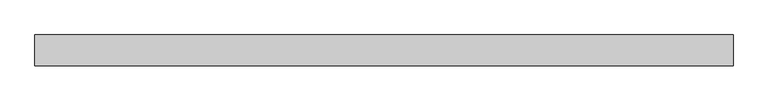
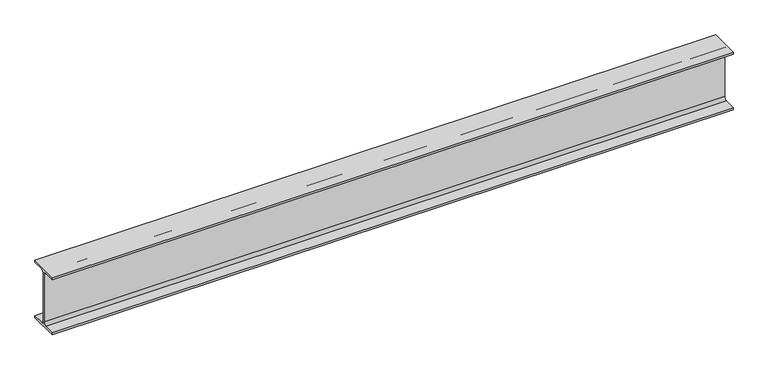
"""IFC4 building model written with IfcOpenShell, lengths in millimetres: beam geometry, 0912_Steel Framing_H-KSD3502 : H_SB_ASB_H-250x125x6x9."""

import ifcopenshell
import ifcopenshell.guid

model = None  # the IFC model being written
_history = None  # IfcOwnerHistory: only IFC2X3 demands one
_inside = {}  # id of a spatial element -> (the spatial element, [elements in it])
_under = {}  # id of a project, library or spatial element -> (it, [spatial elements below it])
_declared = {}  # id of a project -> (the project, [libraries it declares])
_typed = {}  # id of a type object -> (the type object, [elements of that type])
_made_of = {}  # id of a material, layer set ... -> (it, [elements and type objects made of it])


def new_model(schema):
    """Start an empty IFC model of exactly this schema.

    Asked for "IFC4X3", IfcOpenShell would pick the latest addendum, in which some entities
    have other attributes; the version numbers below select the first issue.
    IFC2X3 requires an IfcOwnerHistory on every rooted entity: one is made here for all.
    """
    global model, _history
    if schema == "IFC4X3":
        model = ifcopenshell.file(schema_version=(4, 3, 0, 0))
    else:
        model = ifcopenshell.file(schema=schema)
    _inside.clear()
    _under.clear()
    _declared.clear()
    _typed.clear()
    _made_of.clear()
    _history = None
    if model.schema == "IFC2X3":
        org = make("IfcOrganization", Name="unknown")
        user = make(
            "IfcPersonAndOrganization",
            ThePerson=make("IfcPerson", FamilyName="unknown"),
            TheOrganization=org,
        )
        app = make(
            "IfcApplication",
            ApplicationDeveloper=org,
            Version="unknown",
            ApplicationFullName="unknown",
            ApplicationIdentifier="unknown",
        )
        _history = make(
            "IfcOwnerHistory",
            OwningUser=user,
            OwningApplication=app,
            ChangeAction="ADDED",
            CreationDate=0,
        )
    return model


def make(cls, **values):
    """One entity of the class cls with the attributes given. An attribute that is None is left unset."""
    return model.create_entity(
        cls, **{name: value for name, value in values.items() if value is not None}
    )


def rooted(cls, **values):
    """An entity with a GlobalId (a new one), such as an element, a storey or a relation."""
    return make(cls, GlobalId=ifcopenshell.guid.new(), OwnerHistory=_history, **values)


def si_unit(unit_type, name, prefix=None):
    """IfcSIUnit, for example si_unit("LENGTHUNIT", "METRE", prefix="MILLI")."""
    return make("IfcSIUnit", UnitType=unit_type, Prefix=prefix, Name=name)


def assignment(units):
    """IfcUnitAssignment: the units of a project."""
    return None if units is None else make("IfcUnitAssignment", Units=units)


def point(xyz):
    """IfcCartesianPoint."""
    return None if xyz is None else make("IfcCartesianPoint", Coordinates=xyz)


def direction(xyz):
    """IfcDirection."""
    return None if xyz is None else make("IfcDirection", DirectionRatios=xyz)


def frame(location, z_axis=None, x_axis=None):
    """IfcAxis2Placement3D, a coordinate frame: its origin and axes. An axis left out is left unset."""
    return make(
        "IfcAxis2Placement3D",
        Location=point(location),
        Axis=direction(z_axis),
        RefDirection=direction(x_axis),
    )


def frame_2d(location, x_axis=None):
    """IfcAxis2Placement2D, a coordinate frame in the plane: its origin and x axis."""
    return make(
        "IfcAxis2Placement2D", Location=point(location), RefDirection=direction(x_axis)
    )


def origin():
    """The frame at (0, 0, 0) with its axes left unset."""
    return frame((0.0, 0.0, 0.0))


def place(relative_to, where):
    """IfcLocalPlacement: puts the frame where relative to a parent placement (None: the world)."""
    return make(
        "IfcLocalPlacement", PlacementRelTo=relative_to, RelativePlacement=where
    )


def context(
    kind, dimensions, precision=None, world=None, true_north=None, identifier=None
):
    """IfcGeometricRepresentationContext, for example the 3D "Model" context."""
    return make(
        "IfcGeometricRepresentationContext",
        ContextIdentifier=identifier,
        ContextType=kind,
        CoordinateSpaceDimension=dimensions,
        Precision=precision,
        WorldCoordinateSystem=world,
        TrueNorth=true_north,
    )


def project(units=None, contexts=None):
    """IfcProject with its units and contexts."""
    return rooted(
        "IfcProject",
        Name="project",
        RepresentationContexts=contexts,
        UnitsInContext=assignment(units),
    )


def spatial(cls, under=None, at=None, **own):
    """A site, building, storey or space (cls), placed at a placement, below another one or the project."""
    s = rooted(cls, ObjectPlacement=at, **own)
    if under is not None:
        _under.setdefault(under.id(), (under, []))[1].append(s)
    return s


def polyline(points):
    """IfcPolyline through the points."""
    return make("IfcPolyline", Points=[point(p) for p in points])


def circle_curve(where, radius):
    """IfcCircle in the frame where."""
    return make("IfcCircle", Position=where, Radius=radius)


def trimmed(basis, trim1, trim2, sense, master):
    """IfcTrimmedCurve: the piece of a basis curve between two trims."""
    return make(
        "IfcTrimmedCurve",
        BasisCurve=basis,
        Trim1=trim1,
        Trim2=trim2,
        SenseAgreement=sense,
        MasterRepresentation=master,
    )


def segment(curve, same_sense, transition):
    """IfcCompositeCurveSegment."""
    return make(
        "IfcCompositeCurveSegment",
        Transition=transition,
        SameSense=same_sense,
        ParentCurve=curve,
    )


def composite_curve(segments, self_intersect=None):
    """IfcCompositeCurve: segments joined end to end."""
    return make("IfcCompositeCurve", Segments=segments, SelfIntersect=self_intersect)


def outline(outer, holes=None, kind="AREA"):
    """IfcArbitraryClosedProfileDef: a profile drawn as a closed curve; with holes, ...WithVoids."""
    if holes is None:
        return make("IfcArbitraryClosedProfileDef", ProfileType=kind, OuterCurve=outer)
    return make(
        "IfcArbitraryProfileDefWithVoids",
        ProfileType=kind,
        OuterCurve=outer,
        InnerCurves=holes,
    )


def extrude(swept, where, along, depth):
    """IfcExtrudedAreaSolid: the profile swept, set in the frame where, extruded along a direction by depth."""
    return make(
        "IfcExtrudedAreaSolid",
        SweptArea=swept,
        Position=where,
        ExtrudedDirection=direction(along),
        Depth=depth,
    )


def shape(context_of_items, identifier, shape_type, items):
    """IfcShapeRepresentation: the items that make up one representation, for example the "Body"."""
    return make(
        "IfcShapeRepresentation",
        ContextOfItems=context_of_items,
        RepresentationIdentifier=identifier,
        RepresentationType=shape_type,
        Items=items,
    )


def source(mapping_origin, context_of_items, identifier, shape_type, items):
    """IfcRepresentationMap: a shape defined once, which mapped items show again and again."""
    return make(
        "IfcRepresentationMap",
        MappingOrigin=mapping_origin,
        MappedRepresentation=shape(context_of_items, identifier, shape_type, items),
    )


def transform(
    local_origin,
    x_axis=None,
    y_axis=None,
    z_axis=None,
    scale=None,
    scale2=None,
    scale3=None,
    uniform=True,
):
    """IfcCartesianTransformationOperator3D, or its non-uniform kind. x_axis, y_axis, z_axis: its Axis1, 2, 3."""
    if uniform:
        return make(
            "IfcCartesianTransformationOperator3D",
            Axis1=direction(x_axis),
            Axis2=direction(y_axis),
            LocalOrigin=point(local_origin),
            Scale=scale,
            Axis3=direction(z_axis),
        )
    return make(
        "IfcCartesianTransformationOperator3DnonUniform",
        Axis1=direction(x_axis),
        Axis2=direction(y_axis),
        LocalOrigin=point(local_origin),
        Scale=scale,
        Axis3=direction(z_axis),
        Scale2=scale2,
        Scale3=scale3,
    )


def mapped(mapping_source, mapping_target):
    """IfcMappedItem: shows the shape of a source again, moved by a transform."""
    return make(
        "IfcMappedItem", MappingSource=mapping_source, MappingTarget=mapping_target
    )


def made_of(thing, what):
    """Note that an element or type object is made of a material, layer set ...; save() writes the relation."""
    if what is not None:
        _made_of.setdefault(what.id(), (what, []))[1].append(thing)
    return thing


def element(
    cls,
    number,
    at=None,
    inside=None,
    cuts=None,
    type_object=None,
    material=None,
    context=None,
    identifier="Body",
    shape_type=None,
    held_by="IfcProductDefinitionShape",
    body=None,
    shapes=None,
    **own,
):
    """One element of the class cls, such as IfcWall. Its Tag is "e" and its number.

    at: its placement. inside: the storey or other place that contains it. cuts: it is an
    opening in that element (IfcRelVoidsElement). A single representation is given by context,
    identifier, shape_type and body (its items); several are given by shapes. held_by: the class
    of the entity that holds the representations. save() writes the other relations.
    """
    e = rooted(cls, Tag="e%d" % number, ObjectPlacement=at, **own)
    if body is not None:
        shapes = [shape(context, identifier, shape_type, body)]
    if shapes is not None:
        e.Representation = make(held_by, Representations=shapes)
    if inside is not None:
        _inside.setdefault(inside.id(), (inside, []))[1].append(e)
    if cuts is not None:
        rooted(
            "IfcRelVoidsElement", RelatingBuildingElement=cuts, RelatedOpeningElement=e
        )
    if type_object is not None:
        _typed.setdefault(type_object.id(), (type_object, []))[1].append(e)
    return made_of(e, material)


def aggregate(whole, parts):
    """IfcRelAggregates: a whole, such as a stair, and the parts it consists of."""
    return rooted("IfcRelAggregates", RelatingObject=whole, RelatedObjects=parts)


def save(model, path):
    """Write the relations noted so far, then the file.

    IfcRelAggregates (storeys below a building ...), IfcRelContainedInSpatialStructure (elements
    in a storey), IfcRelDefinesByType, IfcRelAssociatesMaterial and IfcRelDeclares: one each for
    every whole, place, type object, material and project.
    """
    for whole, parts in _under.values():
        aggregate(whole, parts)
    for where, things in _inside.values():
        rooted(
            "IfcRelContainedInSpatialStructure",
            RelatedElements=things,
            RelatingStructure=where,
        )
    for kind, things in _typed.values():
        rooted("IfcRelDefinesByType", RelatedObjects=things, RelatingType=kind)
    for what, things in _made_of.values():
        rooted("IfcRelAssociatesMaterial", RelatedObjects=things, RelatingMaterial=what)
    for by, libraries in _declared.values():
        rooted("IfcRelDeclares", RelatingContext=by, RelatedDefinitions=libraries)
    model.write(path)


def beam_e570f850(model_context):
    return source(origin(), model_context, "Body", "SweptSolid", [
        extrude(outline(composite_curve([segment(polyline([(62.5, -116.0), (62.5, -125.0), (-62.5, -125.0), (-62.5, -116.0), (-15.0, -116.0)]), True, "CONTINUOUS"), segment(trimmed(circle_curve(frame_2d((-15.0, -104.0)), 12.0), [point((-15.0, -116.0))], [point((-3.0, -104.0))], True, "CARTESIAN"), True, "CONTINUOUS"), segment(polyline([(-3.0, -104.0), (-3.0, 104.0)]), True, "CONTINUOUS"), segment(trimmed(circle_curve(frame_2d((-15.0, 104.0)), 12.0), [point((-3.0, 104.0))], [point((-15.0, 116.0))], True, "CARTESIAN"), True, "CONTINUOUS"), segment(polyline([(-15.0, 116.0), (-62.5, 116.0), (-62.5, 125.0), (62.5, 125.0), (62.5, 116.0), (15.0, 116.0)]), True, "CONTINUOUS"), segment(trimmed(circle_curve(frame_2d((15.0, 104.0)), 12.0), [point((15.0, 116.0))], [point((3.0, 104.0))], True, "CARTESIAN"), True, "CONTINUOUS"), segment(polyline([(3.0, 104.0), (3.0, -104.0)]), True, "CONTINUOUS"), segment(trimmed(circle_curve(frame_2d((15.0, -104.0)), 12.0), [point((3.0, -104.0))], [point((15.0, -116.0))], True, "CARTESIAN"), True, "CONTINUOUS"), segment(polyline([(15.0, -116.0), (62.5, -116.0)]), True, "CONTINUOUS")], self_intersect=False)), frame((-1404.8000503, 0.0, 0.0), z_axis=(1.0, 0.0, 0.0), x_axis=(0.0, 1.0, 0.0)), (0.0, 0.0, 1.0), 2809.5192866),
    ])


if __name__ == "__main__":
    model = new_model("IFC4")
    model_context = context("Model", 3, world=origin())
    ifc_project = project(units=[si_unit("LENGTHUNIT", "METRE", prefix="MILLI")], contexts=[model_context])
    site = spatial("IfcSite", under=ifc_project)
    building = spatial("IfcBuilding", under=site)
    placement = place(None, origin())
    beam_shape = beam_e570f850(model_context)
    element("IfcBeam", 1, ObjectType="0912_Steel Framing_H-KSD3502 : H_SB_ASB_H-250x125x6x9", at=placement, inside=building, context=model_context, shape_type="MappedRepresentation", body=[
        mapped(beam_shape, transform((0.0, 0.0, 0.0), x_axis=(1.0, 0.0, 0.0), y_axis=(0.0, 1.0, 0.0), z_axis=(0.0, 0.0, 1.0))),
    ])
    save(model, "model.ifc")

# Revit data of these elements
# Type "0912_Steel Framing_H-KSD3502 : H_SB_ASB_H-250x125x6x9"
#   H_WM Code_1 = "S01AA003-00001 | Main Steel Structure Fabrication Work | Shelter/Building | Light Steel - Standard (30KG/M>Weight) | Material: (   )"
#   H_WM Code_2 = "S03AA029-00001 | Main Steel Structure Erection Work | Shelter/Building | Light Steel (30KG/M>Weight) | Material: (   )"
#   H_WM Code_3 = "S01AA010-00001 | Main Steel Structure Fabrication Work | Shelter/Building | Steel Painting/Coating | for Non-Fireproofed Steel Surface, Surface Preparation, Primer, Second & Final Coat | Material: (   )"
#   H_Q'ty Cal Type Tag = "SB-Q2"
#   Width = 12.5 cm
#   Web Thickness = 0.6 cm
#   Web Fillet = 1.2 cm
#   Warping Constant = 42539.8 cm⁶
#   W = 0
#   Torsional Moment of Inertia = 7.8102 cm⁴
#   Section Area = 37.66 cm²
#   Plastic Modulus weak axis = 73.1 cm³
#   Plastic Modulus strong axis = 366.0 cm³
#   Perimeter = 0.97 m²/m
#   Nominal Weight = 29.60 kgf/m
#   Moment of Inertia weak axis = 294.00 cm⁴
#   Moment of Inertia strong axis = 4050.00 cm⁴
#   Height = 25.0 cm
#   Flange Thickness = 0.9 cm
#   Elastic Modulus weak axis = 47.0 cm³
#   Elastic Modulus strong axis = 324.0 cm³
#   Centroid Vertical = 12.5 cm
#   Centroid Horizontal = 6.25 cm
#   Ix = 40500000
#   Length [instance default] = 1.5240 m
#   Zx = 366000
#   b = 0.1250 m
#   h = 0.2500 m
#   r = 0.0120 m
#   s = 0.0060 m
#   t = 0.0090 m
#   A = 0.003766 m²
#   Structural Material [instance default] = Steel, 45-345
#   Assembly Code = ""
# Element 1 (IfcBeam, "0912_Steel Framing_H-KSD3502 : H_SB_ASB_H-250x125x6x9")
#   Structural Material = none
# Materials
#   "Steel, 45-345": class "Metal", colour RGB 189 187 185, transparency 0, Description = "Steel 345 MPa", Cost = 0
